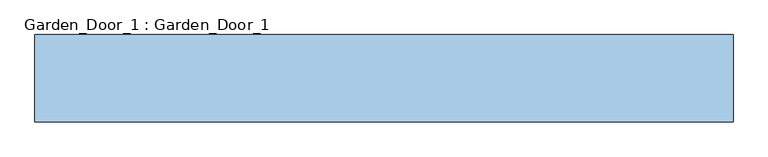
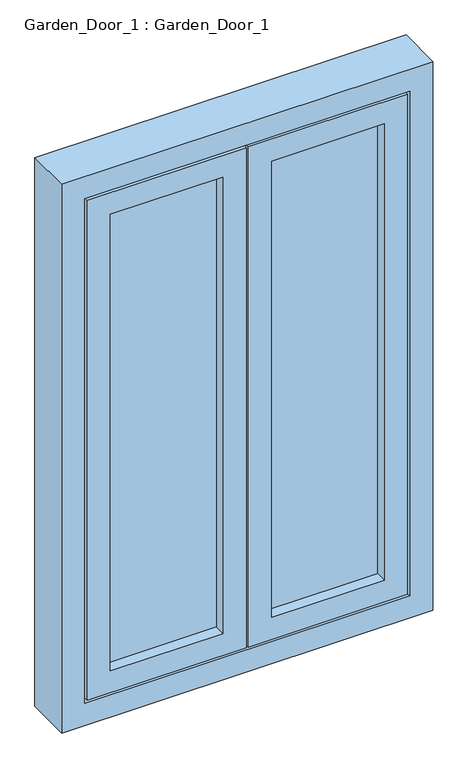
"""IFC4 building model written with IfcOpenShell, lengths in millimetres: window geometry, Garden_Door_1 : Garden_Door_1."""

from ifc_helpers import new_model, si_unit, frame, origin, place, context, project, spatial, polyline, outline, extrude, source, transform, mapped, element, save


def garden_door_1_garden_door_1_5a744e37(model_context):
    return source(origin(), model_context, "Body", "SweptSolid", [
        extrude(outline(polyline([(1355.0, 16765.0), (1840.0, 16765.0), (1840.0, 16755.0), (1355.0, 16755.0), (1355.0, 16765.0)])), frame((0.0, 0.0, 460.0), z_axis=(0.0, 0.0, 1.0), x_axis=(1.0, 0.0, 0.0)), (0.0, 0.0, 1.0), 2080.0),
        extrude(outline(polyline([(360.0, 1940.0), (2640.0, 1940.0), (2640.0, 1255.0), (360.0, 1255.0), (360.0, 1940.0)]), holes=[polyline([(460.0, 1355.0), (2540.0, 1355.0), (2540.0, 1840.0), (460.0, 1840.0), (460.0, 1355.0)])]), frame((0.0, 16705.0, 0.0), z_axis=(0.0, 1.0, 0.0), x_axis=(0.0, 0.0, 1.0)), (0.0, 0.0, 1.0), 100.0),
        extrude(outline(polyline([(660.0, 16765.0), (1145.0, 16765.0), (1145.0, 16755.0), (660.0, 16755.0), (660.0, 16765.0)])), frame((0.0, 0.0, 460.0), z_axis=(0.0, 0.0, 1.0), x_axis=(1.0, 0.0, 0.0)), (0.0, 0.0, 1.0), 2080.0),
        extrude(outline(polyline([(360.0, 1245.0), (2640.0, 1245.0), (2640.0, 560.0), (360.0, 560.0), (360.0, 1245.0)]), holes=[polyline([(460.0, 660.0), (2540.0, 660.0), (2540.0, 1145.0), (460.0, 1145.0), (460.0, 660.0)])]), frame((0.0, 16705.0, 0.0), z_axis=(0.0, 1.0, 0.0), x_axis=(0.0, 0.0, 1.0)), (0.0, 0.0, 1.0), 100.0),
        extrude(outline(polyline([(250.0, 2050.0), (2750.0, 2050.0), (2750.0, 450.0), (250.0, 450.0), (250.0, 2050.0)]), holes=[polyline([(350.0, 550.0), (2650.0, 550.0), (2650.0, 1950.0), (350.0, 1950.0), (350.0, 550.0)])]), frame((0.0, 16705.0, 0.0), z_axis=(0.0, 1.0, 0.0), x_axis=(0.0, 0.0, 1.0)), (0.0, 0.0, 1.0), 200.0),
    ])


if __name__ == "__main__":
    model = new_model("IFC4")
    model_context = context("Model", 3, world=origin())
    ifc_project = project(units=[si_unit("LENGTHUNIT", "METRE", prefix="MILLI")], contexts=[model_context])
    site = spatial("IfcSite", under=ifc_project)
    building = spatial("IfcBuilding", under=site)
    placement = place(None, origin())
    garden_door_1_garden_door_1_shape = garden_door_1_garden_door_1_5a744e37(model_context)
    element("IfcWindow", 1, ObjectType="Garden_Door_1 : Garden_Door_1", at=placement, inside=building, context=model_context, shape_type="MappedRepresentation", body=[
        mapped(garden_door_1_garden_door_1_shape, transform((0.0, 0.0, 0.0), x_axis=(1.0, 0.0, 0.0), y_axis=(0.0, 1.0, 0.0), z_axis=(0.0, 0.0, 1.0))),
    ])
    save(model, "model.ifc")

# Revit data of these elements
# Type "Garden_Door_1 : Garden_Door_1"
#   Type Mark = "50"
#   NameOverride = "Garden_Door_1"
# Element 1 (IfcWindow, "Garden_Door_1 : Garden_Door_1")
#   Materials on its faces: "IfcSurfaceStyle #392", "IfcSurfaceStyle #398"
# Materials
#   "IfcSurfaceStyle #392": class "Unassigned", colour RGB 204 204 204, transparency 0
#   "IfcSurfaceStyle #398": class "Unassigned", colour RGB 93 183 203, transparency 0.85
